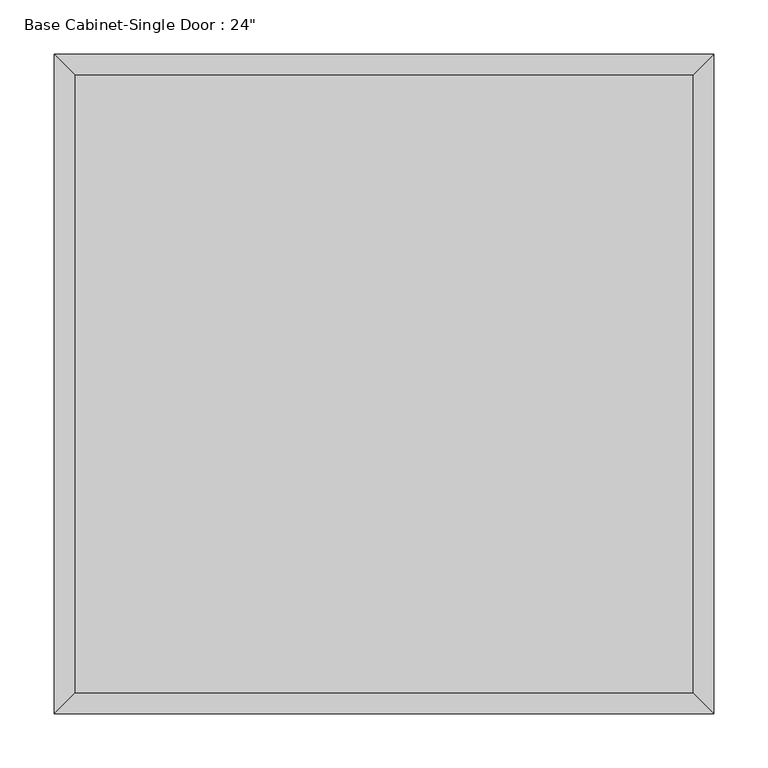
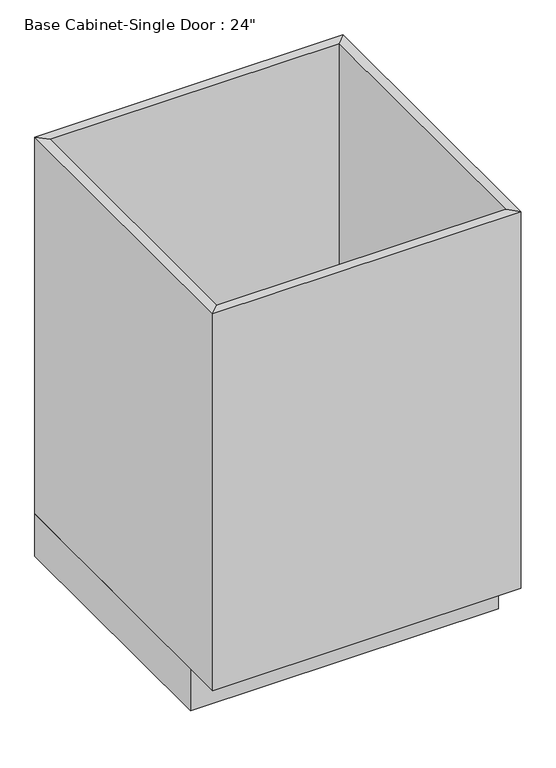
"""IFC4 building model written with IfcOpenShell, lengths in millimetres: furniture geometry."""

from ifc_helpers import new_model, si_unit, frame, origin, origin_with_axes, place, context, project, spatial, polyline, outline, extrude, faceted_brep, source, transform, mapped, element, save


def furniture_222d96cf(model_context):
    return source(origin(), model_context, "Body", "SolidModel", [
        extrude(outline(polyline([(304.4877049, -19.05), (304.4877049, -590.55), (-267.0122951, -590.55), (-267.0122951, -19.05), (304.4877049, -19.05)])), frame((0.0, 0.0, 88.9), z_axis=(0.0, 0.0, 1.0), x_axis=(1.0, 0.0, 0.0)), (0.0, 0.0, 1.0), 19.05),
        faceted_brep([(304.4877049, -590.55, 876.3), (304.4877049, -590.55, 88.9), (-267.0122951, -590.55, 88.9), (-267.0122951, -590.55, 876.3), (323.5377049, -609.6, 876.3), (-286.0622951, -609.6, 876.3), (323.5377049, -609.6, 88.9), (-286.0622951, -609.6, 88.9), (-267.0122951, -19.05, 88.9), (-267.0122951, -19.05, 876.3), (-286.0622951, 0.0, 876.3), (-286.0622951, 0.0, 88.9), (304.4877049, -19.05, 88.9), (304.4877049, -19.05, 876.3), (323.5377049, 0.0, 876.3), (323.5377049, 0.0, 88.9)], [[[0, 1, 2, 3]], [[4, 0, 3, 5]], [[6, 4, 5, 7]], [[1, 6, 7, 2]], [[3, 2, 8, 9]], [[5, 3, 9, 10]], [[7, 5, 10, 11]], [[2, 7, 11, 8]], [[9, 8, 12, 13]], [[10, 9, 13, 14]], [[11, 10, 14, 15]], [[8, 11, 15, 12]], [[13, 12, 1, 0]], [[14, 13, 0, 4]], [[15, 14, 4, 6]], [[12, 15, 6, 1]]]),
        extrude(outline(polyline([(323.5377049, 0.0), (323.5377049, -533.4), (-286.0622951, -533.4), (-286.0622951, 0.0), (323.5377049, 0.0)])), origin_with_axes(), (0.0, 0.0, 1.0), 88.9),
    ])


if __name__ == "__main__":
    model = new_model("IFC4")
    model_context = context("Model", 3, world=origin())
    ifc_project = project(units=[si_unit("LENGTHUNIT", "METRE", prefix="MILLI")], contexts=[model_context])
    site = spatial("IfcSite", under=ifc_project)
    building = spatial("IfcBuilding", under=site)
    placement = place(None, origin())
    furniture_shape = furniture_222d96cf(model_context)
    element("IfcFurniture", 1, ObjectType="Base Cabinet-Single Door : 24\"", at=placement, inside=building, context=model_context, shape_type="MappedRepresentation", body=[
        mapped(furniture_shape, transform((0.0, 0.0, 0.0), x_axis=(1.0, 0.0, 0.0), y_axis=(0.0, 1.0, 0.0), z_axis=(0.0, 0.0, 1.0))),
    ])
    save(model, "model.ifc")

# Revit data of these elements
# Type "Base Cabinet-Single Door : 24\""
#   Depth = 2' - 0"
#   Height = 2' - 10 1/2"
#   Toe Depth = 0' - 3"
#   Toe Height = 0' - 3 1/2"
#   Width = 2' - 0"
# Element 1 (IfcFurniture, "Base Cabinet-Single Door : 24\"")
#   Materials on its faces: "Cabinet"
# Materials
#   "Cabinet": class "Wood", colour RGB 189 170 130, transparency 0, Cost = 0
